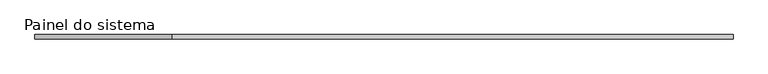
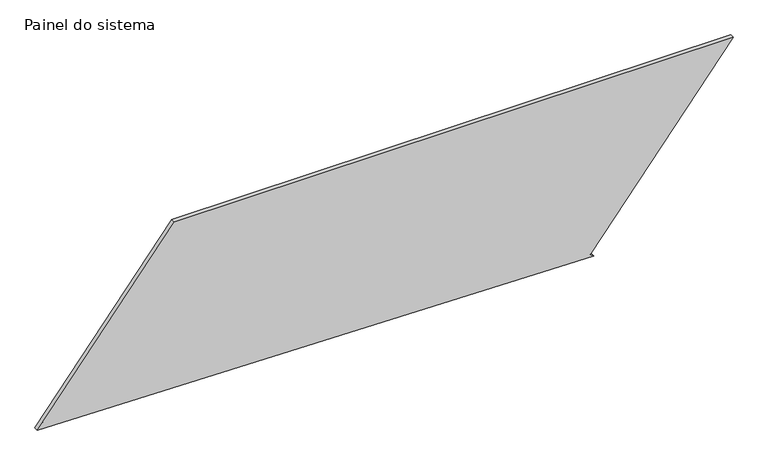
"""IFC4 building model written with IfcOpenShell, lengths in millimetres: plate geometry, Painel do sistema : Envidraçado."""

from ifc_helpers import new_model, si_unit, frame, origin, place, context, project, spatial, polyline, outline, extrude, source, transform, mapped, element, save


def painel_do_sistema_1c6fbe70(model_context):
    return source(origin(), model_context, "Body", "SweptSolid", [
        extrude(outline(polyline([(0.0, 1213.7822157), (15.5601026, 1194.2148141), (1062.606656, 2026.8318434), (1062.606656, -1228.1084412), (58.1825859, -2026.8318434), (0.0, 1213.7822157)])), frame((0.0, 24.5, 0.0), z_axis=(0.0, 1.0, 0.0), x_axis=(0.0, 0.0, 1.0)), (0.0, 0.0, 1.0), 25.0),
    ])


if __name__ == "__main__":
    model = new_model("IFC4")
    model_context = context("Model", 3, world=origin())
    ifc_project = project(units=[si_unit("LENGTHUNIT", "METRE", prefix="MILLI")], contexts=[model_context])
    site = spatial("IfcSite", under=ifc_project)
    building = spatial("IfcBuilding", under=site)
    placement = place(None, origin())
    painel_do_sistema_shape = painel_do_sistema_1c6fbe70(model_context)
    element("IfcPlate", 1, ObjectType="Painel do sistema : Envidraçado", at=placement, inside=building, context=model_context, shape_type="MappedRepresentation", body=[
        mapped(painel_do_sistema_shape, transform((0.0, 0.0, 0.0), x_axis=(1.0, 0.0, 0.0), y_axis=(0.0, 1.0, 0.0), z_axis=(0.0, 0.0, 1.0))),
    ])
    save(model, "model.ifc")

# Revit data of these elements
# Type "Painel do sistema : Envidraçado"
#   Construction Type Id = "GSP4R"
#   Analytic Construction = "Vidraça única Pilkington 1/8 pol"
#   Visual Light Transmittance = 0.9
#   Solar Heat Gain Coefficient = 0.86
#   Heat Transfer Coefficient (U) = 6.7069 W/(m²·K)
# Element 1 (IfcPlate, "Painel do sistema : Envidraçado")
#   Materials on its faces: "Vidro"
# Materials
#   "Vidro": class "Vidro", colour RGB 0 128 192, transparency 0.9, Description = "Vidro de sílica", Cost = 0
